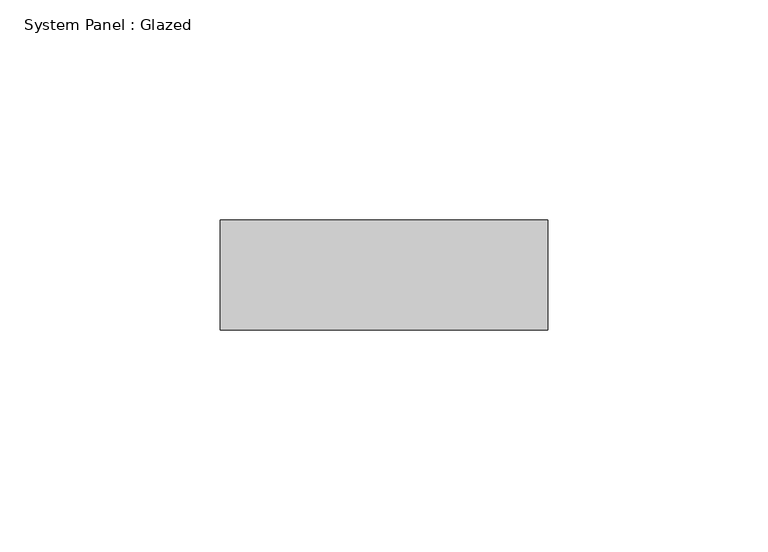
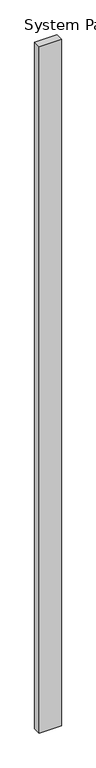
"""IFC4 building model written with IfcOpenShell, lengths in millimetres: plate geometry, System Panel : Glazed."""

from ifc_helpers import new_model, si_unit, origin, origin_with_axes, place, context, project, spatial, polyline, outline, extrude, source, transform, mapped, element, save


def system_panel_glazed_e32ff5c7(model_context):
    return source(origin(), model_context, "Body", "SweptSolid", [
        extrude(outline(polyline([(37.2092572, 24.5), (-37.2092572, 24.5), (-37.2092572, 49.5), (37.2092572, 49.5), (37.2092572, 24.5)])), origin_with_axes(), (0.0, 0.0, 1.0), 2425.0),
    ])


if __name__ == "__main__":
    model = new_model("IFC4")
    model_context = context("Model", 3, world=origin())
    ifc_project = project(units=[si_unit("LENGTHUNIT", "METRE", prefix="MILLI")], contexts=[model_context])
    site = spatial("IfcSite", under=ifc_project)
    building = spatial("IfcBuilding", under=site)
    placement = place(None, origin())
    system_panel_glazed_shape = system_panel_glazed_e32ff5c7(model_context)
    element("IfcPlate", 1, ObjectType="System Panel : Glazed", at=placement, inside=building, context=model_context, shape_type="MappedRepresentation", body=[
        mapped(system_panel_glazed_shape, transform((0.0, 0.0, 0.0), x_axis=(1.0, 0.0, 0.0), y_axis=(0.0, 1.0, 0.0), z_axis=(0.0, 0.0, 1.0))),
    ])
    save(model, "model.ifc")

# Revit data of these elements
# Type "System Panel : Glazed"
#   Keynote = "H11"
#   Construction Type Id = "GSP4R"
#   Analytic Construction = "1/8 in Pilkington single glazing"
#   Visual Light Transmittance = 0.9
#   Solar Heat Gain Coefficient = 0.86
#   Heat Transfer Coefficient (U) = 6.7069 W/(m²·K)
# Element 1 (IfcPlate, "System Panel : Glazed")
#   Materials on its faces: "Glass"
# Materials
#   "Glass": class "Glass", colour RGB 0 128 192, transparency 0.9, Description = "Soda Lime Glass", Cost = 0
